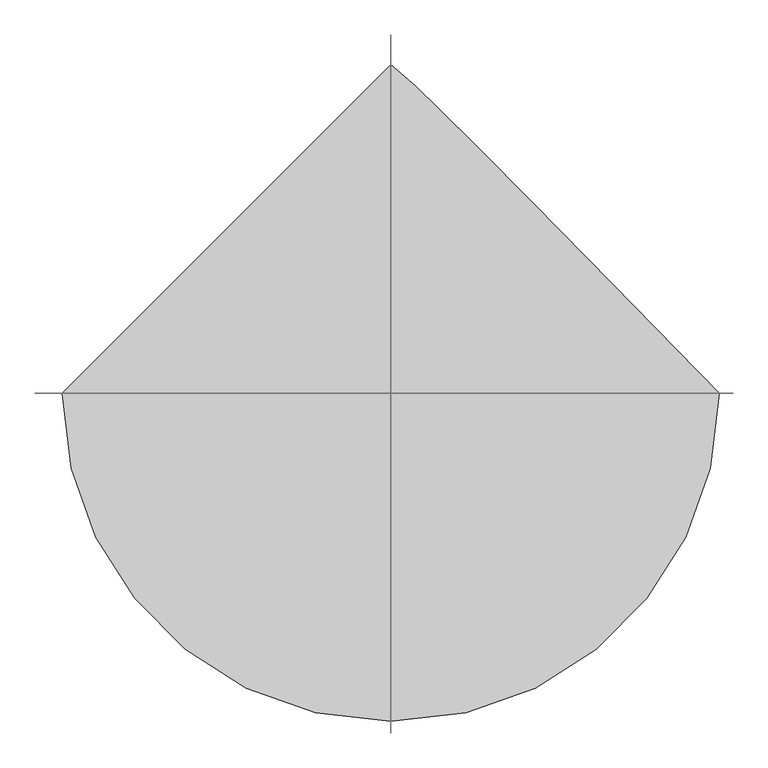
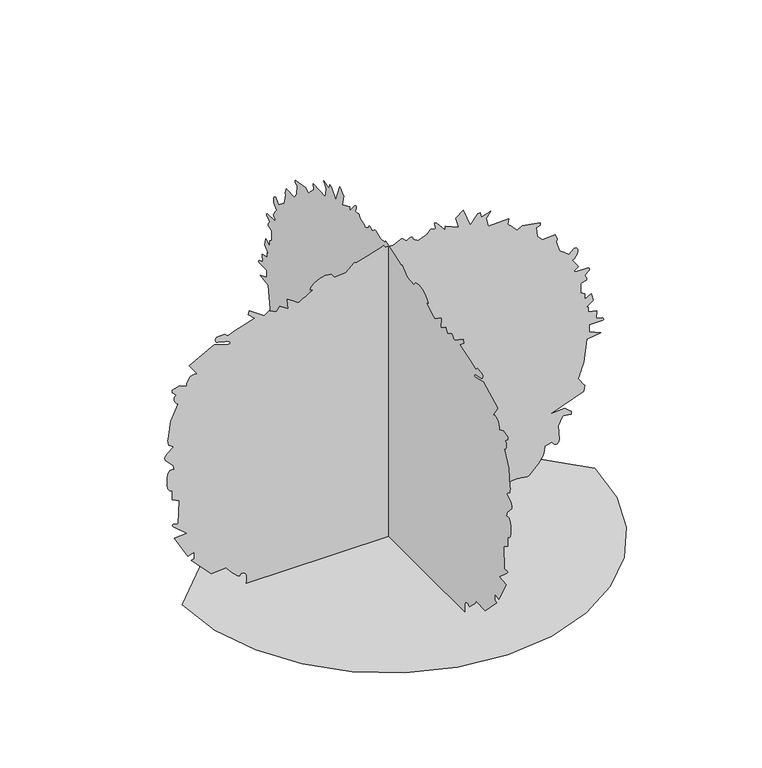
"""IFC4 building model written with IfcOpenShell, lengths in millimetres: proxy geometry, holly 26751 : holly 26751."""

import ifcopenshell
import ifcopenshell.guid

model = None  # the IFC model being written
_history = None  # IfcOwnerHistory: only IFC2X3 demands one
_inside = {}  # id of a spatial element -> (the spatial element, [elements in it])
_under = {}  # id of a project, library or spatial element -> (it, [spatial elements below it])
_declared = {}  # id of a project -> (the project, [libraries it declares])
_typed = {}  # id of a type object -> (the type object, [elements of that type])
_made_of = {}  # id of a material, layer set ... -> (it, [elements and type objects made of it])


def new_model(schema):
    """Start an empty IFC model of exactly this schema.

    Asked for "IFC4X3", IfcOpenShell would pick the latest addendum, in which some entities
    have other attributes; the version numbers below select the first issue.
    IFC2X3 requires an IfcOwnerHistory on every rooted entity: one is made here for all.
    """
    global model, _history
    if schema == "IFC4X3":
        model = ifcopenshell.file(schema_version=(4, 3, 0, 0))
    else:
        model = ifcopenshell.file(schema=schema)
    _inside.clear()
    _under.clear()
    _declared.clear()
    _typed.clear()
    _made_of.clear()
    _history = None
    if model.schema == "IFC2X3":
        org = make("IfcOrganization", Name="unknown")
        user = make(
            "IfcPersonAndOrganization",
            ThePerson=make("IfcPerson", FamilyName="unknown"),
            TheOrganization=org,
        )
        app = make(
            "IfcApplication",
            ApplicationDeveloper=org,
            Version="unknown",
            ApplicationFullName="unknown",
            ApplicationIdentifier="unknown",
        )
        _history = make(
            "IfcOwnerHistory",
            OwningUser=user,
            OwningApplication=app,
            ChangeAction="ADDED",
            CreationDate=0,
        )
    return model


def make(cls, **values):
    """One entity of the class cls with the attributes given. An attribute that is None is left unset."""
    return model.create_entity(
        cls, **{name: value for name, value in values.items() if value is not None}
    )


def rooted(cls, **values):
    """An entity with a GlobalId (a new one), such as an element, a storey or a relation."""
    return make(cls, GlobalId=ifcopenshell.guid.new(), OwnerHistory=_history, **values)


def si_unit(unit_type, name, prefix=None):
    """IfcSIUnit, for example si_unit("LENGTHUNIT", "METRE", prefix="MILLI")."""
    return make("IfcSIUnit", UnitType=unit_type, Prefix=prefix, Name=name)


def assignment(units):
    """IfcUnitAssignment: the units of a project."""
    return None if units is None else make("IfcUnitAssignment", Units=units)


def point(xyz):
    """IfcCartesianPoint."""
    return None if xyz is None else make("IfcCartesianPoint", Coordinates=xyz)


def direction(xyz):
    """IfcDirection."""
    return None if xyz is None else make("IfcDirection", DirectionRatios=xyz)


def frame(location, z_axis=None, x_axis=None):
    """IfcAxis2Placement3D, a coordinate frame: its origin and axes. An axis left out is left unset."""
    return make(
        "IfcAxis2Placement3D",
        Location=point(location),
        Axis=direction(z_axis),
        RefDirection=direction(x_axis),
    )


def origin():
    """The frame at (0, 0, 0) with its axes left unset."""
    return frame((0.0, 0.0, 0.0))


def place(relative_to, where):
    """IfcLocalPlacement: puts the frame where relative to a parent placement (None: the world)."""
    return make(
        "IfcLocalPlacement", PlacementRelTo=relative_to, RelativePlacement=where
    )


def context(
    kind, dimensions, precision=None, world=None, true_north=None, identifier=None
):
    """IfcGeometricRepresentationContext, for example the 3D "Model" context."""
    return make(
        "IfcGeometricRepresentationContext",
        ContextIdentifier=identifier,
        ContextType=kind,
        CoordinateSpaceDimension=dimensions,
        Precision=precision,
        WorldCoordinateSystem=world,
        TrueNorth=true_north,
    )


def project(units=None, contexts=None):
    """IfcProject with its units and contexts."""
    return rooted(
        "IfcProject",
        Name="project",
        RepresentationContexts=contexts,
        UnitsInContext=assignment(units),
    )


def spatial(cls, under=None, at=None, **own):
    """A site, building, storey or space (cls), placed at a placement, below another one or the project."""
    s = rooted(cls, ObjectPlacement=at, **own)
    if under is not None:
        _under.setdefault(under.id(), (under, []))[1].append(s)
    return s


def point_list(points):
    """IfcCartesianPointList2D or 3D."""
    cls = (
        "IfcCartesianPointList2D" if len(points[0]) == 2 else "IfcCartesianPointList3D"
    )
    return make(cls, CoordList=points)


def triangles(points, corners, closed=None, point_numbers=None):
    """IfcTriangulatedFaceSet: each triangle names its three corners, points numbered from 1."""
    return make(
        "IfcTriangulatedFaceSet",
        Coordinates=point_list(points),
        Closed=closed,
        CoordIndex=corners,
        PnIndex=point_numbers,
    )


def shape(context_of_items, identifier, shape_type, items):
    """IfcShapeRepresentation: the items that make up one representation, for example the "Body"."""
    return make(
        "IfcShapeRepresentation",
        ContextOfItems=context_of_items,
        RepresentationIdentifier=identifier,
        RepresentationType=shape_type,
        Items=items,
    )


def source(mapping_origin, context_of_items, identifier, shape_type, items):
    """IfcRepresentationMap: a shape defined once, which mapped items show again and again."""
    return make(
        "IfcRepresentationMap",
        MappingOrigin=mapping_origin,
        MappedRepresentation=shape(context_of_items, identifier, shape_type, items),
    )


def transform(
    local_origin,
    x_axis=None,
    y_axis=None,
    z_axis=None,
    scale=None,
    scale2=None,
    scale3=None,
    uniform=True,
):
    """IfcCartesianTransformationOperator3D, or its non-uniform kind. x_axis, y_axis, z_axis: its Axis1, 2, 3."""
    if uniform:
        return make(
            "IfcCartesianTransformationOperator3D",
            Axis1=direction(x_axis),
            Axis2=direction(y_axis),
            LocalOrigin=point(local_origin),
            Scale=scale,
            Axis3=direction(z_axis),
        )
    return make(
        "IfcCartesianTransformationOperator3DnonUniform",
        Axis1=direction(x_axis),
        Axis2=direction(y_axis),
        LocalOrigin=point(local_origin),
        Scale=scale,
        Axis3=direction(z_axis),
        Scale2=scale2,
        Scale3=scale3,
    )


def mapped(mapping_source, mapping_target):
    """IfcMappedItem: shows the shape of a source again, moved by a transform."""
    return make(
        "IfcMappedItem", MappingSource=mapping_source, MappingTarget=mapping_target
    )


def made_of(thing, what):
    """Note that an element or type object is made of a material, layer set ...; save() writes the relation."""
    if what is not None:
        _made_of.setdefault(what.id(), (what, []))[1].append(thing)
    return thing


def element(
    cls,
    number,
    at=None,
    inside=None,
    cuts=None,
    type_object=None,
    material=None,
    context=None,
    identifier="Body",
    shape_type=None,
    held_by="IfcProductDefinitionShape",
    body=None,
    shapes=None,
    **own,
):
    """One element of the class cls, such as IfcWall. Its Tag is "e" and its number.

    at: its placement. inside: the storey or other place that contains it. cuts: it is an
    opening in that element (IfcRelVoidsElement). A single representation is given by context,
    identifier, shape_type and body (its items); several are given by shapes. held_by: the class
    of the entity that holds the representations. save() writes the other relations.
    """
    e = rooted(cls, Tag="e%d" % number, ObjectPlacement=at, **own)
    if body is not None:
        shapes = [shape(context, identifier, shape_type, body)]
    if shapes is not None:
        e.Representation = make(held_by, Representations=shapes)
    if inside is not None:
        _inside.setdefault(inside.id(), (inside, []))[1].append(e)
    if cuts is not None:
        rooted(
            "IfcRelVoidsElement", RelatingBuildingElement=cuts, RelatedOpeningElement=e
        )
    if type_object is not None:
        _typed.setdefault(type_object.id(), (type_object, []))[1].append(e)
    return made_of(e, material)


def aggregate(whole, parts):
    """IfcRelAggregates: a whole, such as a stair, and the parts it consists of."""
    return rooted("IfcRelAggregates", RelatingObject=whole, RelatedObjects=parts)


def save(model, path):
    """Write the relations noted so far, then the file.

    IfcRelAggregates (storeys below a building ...), IfcRelContainedInSpatialStructure (elements
    in a storey), IfcRelDefinesByType, IfcRelAssociatesMaterial and IfcRelDeclares: one each for
    every whole, place, type object, material and project.
    """
    for whole, parts in _under.values():
        aggregate(whole, parts)
    for where, things in _inside.values():
        rooted(
            "IfcRelContainedInSpatialStructure",
            RelatedElements=things,
            RelatingStructure=where,
        )
    for kind, things in _typed.values():
        rooted("IfcRelDefinesByType", RelatedObjects=things, RelatingType=kind)
    for what, things in _made_of.values():
        rooted("IfcRelAssociatesMaterial", RelatedObjects=things, RelatingMaterial=what)
    for by, libraries in _declared.values():
        rooted("IfcRelDeclares", RelatingContext=by, RelatedDefinitions=libraries)
    model.write(path)


def entourage_54f20335(model_context):
    return source(origin(), model_context, "Body", "Tessellation", [
        triangles([(-823.0310858, 0.0, 7.21e-05), (-801.2709314, -188.5840741, 7.21e-05), (-739.3050917, -361.7670897, 7.21e-05), (-642.0891506, -514.5912643, 7.21e-05), (-514.5912643, -642.0891506, 7.21e-05), (-361.7670897, -739.3050917, 7.21e-05), (-188.5840741, -801.2709314, 7.21e-05), (3.6e-05, -823.0310858, 7.21e-05), (188.5840741, -801.2709314, 7.21e-05), (361.7670897, -739.3050917, 7.21e-05), (514.5912643, -642.0891506, 7.21e-05), (642.0891506, -514.5912643, 7.21e-05), (739.3050917, -361.7670897, 7.21e-05), (801.2709314, -188.5838197, 7.21e-05), (823.0310858, 7.2e-05, 7.21e-05), (555.5640178, 274.3555465, 7.21e-05), (357.2763754, 476.3515926, 7.21e-05), (216.6411551, 618.0454874, 7.21e-05), (122.1254853, 711.5022102, 7.21e-05), (62.2002777, 768.7766939, 7.21e-05), (25.3349997, 801.933827, 7.21e-05), (-0.0001079, 823.0310858, 7.21e-05), (0.0, 364.688096, 1198.1839863), (0.0, 394.9268025, 1235.9816792), (0.0, 406.2653546, 1235.9816792), (0.0, 410.0448841, 1217.0841408), (0.0, 447.8426133, 1228.4226929), (0.0, 428.9450386, 1205.7430452), (0.0, 436.5040612, 1167.9452797), (0.0, 519.6585786, 1171.727389), (0.0, 515.8790491, 1149.0476686), (0.0, 517.7484844, 1147.6176687), (0.0, 521.9039357, 1143.7644882), (0.0, 527.6798913, 1138.1510954), (0.0, 534.4109121, 1131.4328281), (0.0, 541.4314502, 1124.2699659), (0.0, 548.0735593, 1117.3230789), (0.0, 553.6768147, 1111.2499758), (0.0, 572.5743894, 1122.5885279), (0.0, 644.390391, 1111.2499758), (0.0, 644.390391, 1099.9114237), (0.0, 629.2722731, 1096.1318579), (0.0, 633.0517662, 1058.334165), (0.0, 651.9493773, 1035.6544447), (0.0, 704.8677315, 1039.4340105), (0.0, 712.4267904, 1016.7569063), (0.0, 708.6472973, 1009.1953039), (0.0, 719.9858494, 967.6180452), (0.0, 726.0208735, 963.2238367), (0.0, 732.9550432, 957.9761919), (0.0, 740.1179054, 952.4085085), (0.0, 746.8488899, 947.0389961), (0.0, 752.4800869, 942.3932768), (0.0, 756.345912, 938.9998793), (0.0, 757.7835423, 937.3818821), (0.0, 780.4607191, 956.2794931), (0.0, 789.1297394, 953.9172827), (0.0, 793.4883396, 947.7375), (0.0, 794.1741262, 939.096385), (0.0, 791.8195461, 929.3580259), (0.0, 787.0672199, 919.8812788), (0.0, 780.5495945, 912.0225288), (0.0, 772.9016602, 907.1431755), (0.0, 774.118301, 904.8622828), (-2e-07, 781.5884846, 895.1949949), (-2e-07, 794.0852509, 877.4074179), (0.0, 795.5813078, 873.1249758), (0.0, 794.0014624, 870.5621235), (0.0, 782.7695171, 862.2893), (0.0, 780.9686823, 860.2395704), (0.0, 780.4607191, 858.0068579), (2e-07, 785.7515299, 855.1773067), (-2e-07, 836.9528378, 853.0538898), (0.0, 840.9380596, 850.4453281), (1e-07, 841.2580982, 846.6200529), (1e-07, 839.7290491, 843.1504246), (0.0, 822.0405212, 827.768224), (3e-07, 829.193137, 816.4016939), (5e-07, 829.9424372, 812.9472536), (7e-07, 829.5335232, 809.4446331), (7e-07, 829.7087305, 806.8944981), (6e-07, 827.806303, 805.096134), (0.0, 810.7247875, 799.7900625), (0.0, 806.9198599, 797.5295174), (0.0, 806.9198599, 759.7317518), (0.0, 822.0405212, 748.3931997), (0.0, 822.0405212, 725.7135521), (0.0, 848.4971186, 740.8341408), (0.0, 856.0561775, 710.5954342), (0.0, 829.5995075, 691.6952797), (0.0, 837.1585665, 687.9157866), (0.0, 837.1585665, 669.0181755), (0.0, 871.1767662, 661.4591892), (0.0, 867.3972731, 631.2204826), (-4e-07, 892.5458107, 622.5819111), (-3e-07, 895.9697296, 619.724382), (0.0, 897.6334362, 616.1023647), (3e-07, 893.5719835, 613.0467373), (0.0, 840.9380596, 612.3203281), (0.0, 840.9380596, 582.084165), (0.0, 886.2948841, 563.1840105), (0.0, 829.5995075, 555.6249879), (0.0, 818.258412, 461.1319184), (0.0, 815.0631128, 451.4214646), (0.0, 811.202302, 440.3089889), (0.0, 807.0646185, 428.8484965), (0.0, 803.043861, 418.0966819), (0.0, 799.5284506, 409.1101665), (0.0, 796.9122585, 402.9455718), (0.0, 795.5813078, 400.6545053), (0.0, 820.5621958, 364.3553764), (0.0, 822.0405212, 362.856776), (0.0, 818.258412, 340.1796355), (-1.2e-06, 685.9676497, 291.7393147), (0.0, 742.6629536, 294.8203221), (0.0, 767.2044062, 273.0017229), (0.0, 769.1220943, 272.1432179), (0.0, 769.1220943, 260.8046476), (0.0, 735.1038946, 264.5841771), (0.0, 716.2062836, 230.5654505), (6e-07, 720.5065298, 170.5523622), (4e-07, 718.0097345, 161.443416), (0.0, 712.4267904, 154.9702283), (1e-07, 708.1747971, 154.6016643), (1e-07, 704.4080212, 155.6534715), (1e-07, 701.0399855, 157.7794682), (0.0, 689.7471428, 170.0893091), (0.0, 663.2904728, 162.5297596), (0.0, 661.3549805, 143.989803), (0.0, 655.9651205, 127.1831253), (0.0, 637.3164768, 97.7790698), (0.0, 599.0335665, 60.4761278), (0.0, 593.0747369, 58.4339696), (0.0, 555.4065419, 64.3069578), (0.0, 530.3748576, 63.9444981), (0.0, 505.6580887, 55.865013), (0.0, 484.5938948, 35.9298222), (0.0, 470.5222973, 0.0), (1.9e-06, -527.336998, 0.3946068), (1.9e-06, -526.7324927, 3.4093656), (1.8e-06, -525.6326689, 11.1126779), (1.6e-06, -525.1043581, 21.4932261), (1.4e-06, -526.211776, 32.5396858), (1.3e-06, -530.0217905, 42.240454), (1.2e-06, -537.6011244, 48.584103), (1.1e-06, -550.0141022, 49.5597157), (1.1e-06, -552.9884482, 42.5897014), (9e-07, -560.6973527, 44.5830936), (4e-07, -583.0569617, 64.6592528), (2e-07, -594.0755116, 77.3417272), (1e-07, -602.5667084, 88.1867683), (0.0, -606.7119859, 94.4940959), (0.0, -667.1868193, 90.7143212), (0.0, -746.5618435, 173.8690929), (0.0, -735.2232914, 177.6488585), (0.0, -735.2232914, 204.1070183), (0.0, -761.6799614, 196.547487), (0.0, -814.5983156, 291.0408108), (0.0, -765.461998, 294.8203221), (-1e-07, -818.4387789, 340.9873624), (0.0, -822.1573019, 347.7386945), (-3e-07, -820.8568726, 350.2888295), (-4e-07, -818.2406805, 351.2819738), (0.0, -799.4776543, 347.7386945), (0.0, -795.6981611, 442.2317639), (0.0, -822.1573019, 457.352389), (0.0, -822.1573019, 495.1475747), (0.0, -832.8634071, 498.9677267), (1e-07, -839.8280983, 508.9931322), (2e-07, -843.5822296, 523.0672731), (5e-07, -843.58986, 554.7486969), (7e-07, -840.9076109, 568.0481031), (9e-07, -837.1458492, 576.780637), (6e-07, -835.3424709, 579.5238198), (4e-07, -832.4240444, 581.3678933), (1e-07, -824.7836678, 582.9223406), (0.0, -814.5983156, 582.084165), (0.0, -818.9670897, 599.2621862), (0.0, -850.1633686, 632.368523), (0.0, -852.289329, 643.412471), (0.0, -843.1225193, 657.5323214), (0.0, -818.3778088, 676.5772345), (0.0, -819.0966602, 678.065661), (0.0, -834.2578714, 690.2068531), (0.0, -837.2754198, 691.6952797), (0.0, -841.0549129, 714.375), (0.0, -838.9950096, 718.3525915), (0.0, -829.7163609, 789.9704584), (0.0, -799.4776543, 854.2273647), (0.0, -805.1469303, 855.9037886), (0.0, -809.7265926, 860.3360762), (0.0, -812.954884, 866.6098938), (0.0, -814.5627073, 873.8234797), (0.0, -814.2909216, 881.0700577), (0.0, -811.8703571, 887.4378376), (0.0, -807.0392567, 892.0251303), (0.0, -807.4354534, 892.8607624), (0.0, -812.0837162, 897.9737497), (0.0, -820.8492422, 906.3049999), (0.0, -822.1573019, 907.1431755), (0.0, -822.1573019, 918.4817276), (0.0, -791.9185953, 926.0407866), (0.0, -790.6511581, 925.0044399), (0.0, -777.4609749, 918.7560568), (0.0, -765.461998, 914.7022345), (0.0, -764.4104633, 924.481216), (0.0, -761.392915, 934.0036726), (0.0, -756.6100674, 942.5457384), (0.0, -750.2651785, 949.3884893), (0.0, -742.5613609, 953.8080597), (0.0, -733.6992565, 955.0856707), (0.0, -723.8821959, 952.5), (0.0, -754.1209024, 997.8567518), (0.0, -655.8482672, 1050.775106), (7e-07, -598.9294304, 1033.6808733), (5e-07, -592.5108541, 1034.3742903), (5e-07, -591.6802726, 1035.5045992), (4e-07, -591.6421935, 1037.1784796), (3e-07, -592.2771838, 1039.2003038), (2e-07, -595.0864237, 1043.5360857), (0.0, -599.1504198, 1046.9930695), (0.0, -613.793494, 1050.1477461), (0.0, -641.0578909, 1056.558692), (0.0, -644.5071716, 1058.334165), (1e-07, -646.8948166, 1060.1705355), (1e-07, -648.7185425, 1062.5454632), (1e-07, -649.9529875, 1065.3064138), (1e-07, -650.5574564, 1068.3061581), (0.0, -650.5041166, 1071.3923069), (0.0, -649.7573599, 1074.4174129), (0.0, -648.2892809, 1077.2317034), (-2e-07, -645.2513849, 1079.2662449), (0.0, -614.2710085, 1081.0112692), (0.0, -603.3617543, 1070.5744062), (0.0, -602.9299493, 1069.6727171), (0.0, -567.8931707, 1083.2083735), (0.0, -547.3801423, 1090.3508154), (0.0, -493.3187983, 1107.47041), (0.0, -519.7754319, 1130.1475868), (0.0, -515.9959024, 1145.2681755), (0.0, -455.5210327, 1103.6909168), (0.0, -436.6209146, 1118.8089621), (0.0, -406.382208, 1103.6909168), (0.0, -405.4525772, 1104.4097683), (0.0, -396.018996, 1119.5709795), (0.0, -395.0436559, 1122.5885279), (0.0, -361.0254198, 1099.9114237), (0.0, -365.1427557, 1139.9113077), (0.0, -364.8049493, 1141.4886824), (0.0, -342.607903, 1128.2831657), (0.0, -319.4481611, 1111.2499758), (0.0, -309.9866747, 1116.2283783), (0.0, -299.4278897, 1122.1567228), (0.0, -288.7040166, 1128.4457285), (0.0, -278.7446681, 1134.4934698), (0.0, -270.4795113, 1139.7106659), (0.0, -264.8381769, 1143.5003328), (0.0, -262.752839, 1145.2681755), (0.0, -273.3471778, 1149.5912401), (0.0, -269.0418629, 1159.9925674), (0.0, -254.1727123, 1172.6036436), (0.0, -233.0803043, 1183.5662739), (0.0, -210.0991489, 1189.0196474), (0.0, -189.5657729, 1185.1004826), (0.0, -175.8177748, 1167.9452797), (0.0, -130.4607414, 1171.727389), (0.0, -96.4430322, 1201.9634794), (0.0, -95.7204019, 1201.8238077), (0.0, -89.6495515, 1198.8037886), (0.0, -88.8834827, 1198.1839863), (0.0, -39.7464248, 1213.3046476), (0.0, 20.7297008, 1232.2022587), (0.0, 21.3109812, 1231.442712), (0.0, 21.9957141, 1230.3632721), (0.0, 22.7131871, 1229.0906754), (0.0, 23.3937551, 1227.7547104), (0.0, 23.9666262, 1226.4821136), (0.0, 24.3619509, 1225.4026737), (0.0, 24.5094506, 1224.6431271), (0.0, 58.527187, 1220.8637066), (0.0, 88.228163, 1235.3035229), (0.0, 92.5451506, 1235.9816792), (-1e-07, 95.4963785, 1234.686264), (0.0, 109.5573117, 1221.6231079), (0.0, 111.4440243, 1220.8637066), (0.0, 122.4526365, 1227.7801449), (0.0, 128.2821862, 1229.7790054), (0.0, 133.4833494, 1229.5072197), (0.0, 137.0317248, 1225.6972778), (0.0, 137.9024383, 1217.0841408), (0.0, 140.9202138, 1215.7049372), (0.0, 144.3867991, 1213.9269207), (0.0, 147.9687116, 1211.9380886), (0.0, 151.3339586, 1209.9340685), (0.0, 154.1492937, 1208.1052557), (0.0, 156.0827331, 1206.6447344), (0.0, 156.801312, 1205.7430452), (0.0, 162.3971732, 1208.1433348), (0.0, 169.0263289, 1210.9119158), (0.0, 176.0290991, 1213.7770752), (0.0, 182.746894, 1216.4745123), (0.0, 188.5205787, 1218.7325867), (0.0, 192.691, 1220.2871429), (0.0, 194.5987869, 1220.8637066), (0.0, 205.4400219, 1235.8141022), (0.0, 205.9381202, 1235.9816792), (0.0, 208.316318, 1235.3645657), (0.0, 227.1496525, 1232.3444012), (0.0, 228.6167504, 1232.2022587), (1e-07, 223.3642912, 1249.3599323), (1e-07, 222.9002389, 1253.4188416), (1e-07, 223.3033211, 1256.642046), (0.0, 224.8369848, 1258.6613995), (-3e-07, 231.8636453, 1254.2900093), (0.0, 264.139673, 1215.5067661), (0.0, 266.4129717, 1213.3046476), (0.0, 266.4129717, 1228.4226929), (0.0, 319.3313441, 1205.7430452), (0.0, 307.9927557, 1247.3202312), (0.0, 338.2289188, 1269.9999516), (325.0107576, -3.63e-05, 1198.1839863), (355.2494642, -3.85e-05, 1235.9816792), (366.5880163, -3.85e-05, 1235.9816792), (370.3675458, -3.74e-05, 1217.0841408), (408.165275, -3.81e-05, 1228.4226929), (389.2677003, -3.67e-05, 1205.7430452), (396.8267229, -3.44e-05, 1167.9452797), (479.9812403, -3.47e-05, 1171.727389), (476.2017108, -3.33e-05, 1149.0476686), (478.0711461, -3.32e-05, 1147.6176687), (482.2265974, -3.3e-05, 1143.7644882), (488.002553, -3.27e-05, 1138.1510954), (494.7335738, -3.23e-05, 1131.4328281), (501.7515684, -3.18e-05, 1124.2699659), (508.396221, -3.14e-05, 1117.3230789), (513.9994763, -3.11e-05, 1111.2499758), (532.897051, -3.17e-05, 1122.5885279), (604.7130163, -3.11e-05, 1111.2499758), (604.7130163, -3.04e-05, 1099.9114237), (589.5949347, -3.02e-05, 1096.1318579), (593.3744642, -2.79e-05, 1058.334165), (612.2720753, -2.66e-05, 1035.6544447), (665.187886, -2.68e-05, 1039.4340105), (672.7494884, -2.54e-05, 1016.7569063), (668.9699226, -2.5e-05, 1009.1953039), (680.3084747, -2.25e-05, 967.6180452), (686.3434988, -2.22e-05, 963.2238367), (693.2777412, -2.19e-05, 957.9761919), (700.4405308, -2.16e-05, 952.4085085), (707.1715153, -2.13e-05, 947.0389961), (712.8027122, -2.1e-05, 942.3932768), (716.66861, -2.08e-05, 938.9998793), (718.1062403, -2.07e-05, 937.3818821), (740.7833445, -2.18e-05, 956.2794931), (749.4523647, -2.17e-05, 953.9172827), (753.8110376, -2.13e-05, 947.7375), (754.4942808, -2.08e-05, 939.096385), (752.1422441, -2.02e-05, 929.3580259), (747.3899179, -1.97e-05, 919.8812788), (740.8722198, -1.92e-05, 912.0225288), (733.2242855, -1.89e-05, 907.1431755), (734.440999, -1.87e-05, 904.8622828), (741.9111099, -1.8e-05, 895.1949949), (754.4078762, -1.69e-05, 877.4074179), (755.9040058, -1.69e-05, 873.1249758), (754.3240877, -1.68e-05, 870.5621235), (743.0922152, -1.62e-05, 862.2893), (741.2913803, -1.61e-05, 860.2395704), (740.7833445, -1.6e-05, 858.0068579), (746.0741552, -1.6e-05, 855.1773067), (797.2754631, -1.54e-05, 853.0538898), (801.2607576, -1.55e-05, 850.4453281), (801.5807962, -1.54e-05, 846.6200529), (800.0516745, -1.52e-05, 843.1504246), (782.3606031, -1.42e-05, 827.768224), (789.5157623, -1.38e-05, 816.4016939), (790.2650625, -1.38e-05, 812.9472536), (789.8561485, -1.38e-05, 809.4446331), (790.0314285, -1.36e-05, 806.8944981), (788.1289284, -1.34e-05, 805.096134), (771.0474855, -1.25e-05, 799.7900625), (767.2425579, -1.24e-05, 797.5295174), (767.2425579, -1.01e-05, 759.7317518), (782.3606031, -9.4e-06, 748.3931997), (782.3606031, -8.1e-06, 725.7135521), (808.8198166, -9e-06, 740.8341408), (816.3788029, -7.2e-06, 710.5954342), (789.9222055, -6.1e-06, 691.6952797), (797.4812645, -5.8e-06, 687.9157866), (797.4812645, -4.7e-06, 669.0181755), (831.4994642, -4.3e-06, 661.4591892), (827.7198984, -2.5e-06, 631.2204826), (852.8684361, -1.6e-06, 622.5819111), (856.292355, -1.5e-06, 619.724382), (857.9560616, -1.6e-06, 616.1023647), (853.8946089, -1.7e-06, 613.0467373), (801.2607576, -1.3e-06, 612.3203281), (801.2607576, 5e-07, 582.084165), (846.6175095, 1.6e-06, 563.1840105), (789.9222055, 2e-06, 555.6249879), (778.58111, 7.7e-06, 461.1319184), (775.3857382, 8.3e-06, 451.4214646), (771.525, 8.9e-06, 440.3089889), (767.3873165, 9.6e-06, 428.8484965), (763.3664864, 1.02e-05, 418.0966819), (759.8511486, 1.08e-05, 409.1101665), (757.2349566, 1.11e-05, 402.9455718), (755.9040058, 1.13e-05, 400.6545053), (780.8823503, 1.34e-05, 364.3553764), (782.3606031, 1.35e-05, 362.856776), (778.58111, 1.49e-05, 340.1796355), (646.290275, 1.9e-05, 291.7393147), (702.9855789, 1.76e-05, 294.8203221), (727.5271042, 1.89e-05, 273.0017229), (729.4447924, 1.89e-05, 272.1432179), (729.4447924, 1.96e-05, 260.8046476), (695.4265926, 1.94e-05, 264.5841771), (676.5289816, 2.14e-05, 230.5654505), (680.8292278, 2.44e-05, 170.5523622), (678.3323599, 2.51e-05, 161.4436704), (672.7494884, 2.59e-05, 154.9702283), (668.4974951, 2.59e-05, 154.6016643), (664.7306465, 2.58e-05, 155.6534715), (661.3626108, 2.56e-05, 157.7794682), (650.0697681, 2.5e-05, 170.0893091), (623.6106274, 2.55e-05, 162.5297596), (621.675135, 2.66e-05, 143.989803), (616.2852751, 2.76e-05, 127.1833797), (597.6391022, 2.93e-05, 97.7790698), (559.3562282, 3.16e-05, 60.4761278), (553.3948551, 3.17e-05, 58.4342239), (515.7292036, 3.13e-05, 64.3069578), (490.6975193, 3.14e-05, 63.9444981), (465.9807504, 3.18e-05, 55.8652674), (444.9165565, 3.3e-05, 35.9298222), (430.844959, 3.52e-05, 5e-05), (-567.0143363, 3.32e-05, 0.3946575), (-566.409831, 3.31e-05, 3.4094164), (-565.3100072, 3.27e-05, 11.1127279), (-564.7816964, 3.23e-05, 21.4932761), (-565.8891143, 3.18e-05, 32.5396858), (-569.6991288, 3.14e-05, 42.240454), (-577.2784627, 3.11e-05, 48.584103), (-589.6914405, 3.11e-05, 49.5597157), (-592.6657866, 3.16e-05, 42.5897014), (-600.374691, 3.16e-05, 44.5830936), (-622.7343, 3.09e-05, 64.6592528), (-633.7528135, 3.03e-05, 77.3417272), (-642.244083, 2.98e-05, 88.1867683), (-646.3893242, 2.95e-05, 94.4940959), (-706.8641939, 2.98e-05, 90.7143212), (-786.2392181, 2.48e-05, 173.8690929), (-774.900666, 2.46e-05, 177.6488585), (-774.900666, 2.3e-05, 204.1072726), (-801.3598068, 2.35e-05, 196.5477413), (-854.2756176, 1.78e-05, 291.0408108), (-805.1393, 1.76e-05, 294.8203221), (-858.1160809, 1.5e-05, 340.9873624), (-861.8346766, 1.44e-05, 347.7386945), (-860.5341745, 1.46e-05, 350.2888295), (-857.9179825, 1.46e-05, 351.2819738), (-839.1550289, 1.44e-05, 347.7386945), (-835.3754631, 8.8e-06, 442.2317639), (-861.8346766, 7.9e-06, 457.352389), (-861.8346766, 5.7e-06, 495.1475747), (-872.5433252, 5.4e-06, 498.9677267), (-879.5054729, 4.7e-06, 508.9931322), (-883.2595316, 3.8e-06, 523.0672731), (-883.2671619, 1.6e-06, 554.7486969), (-880.5874563, 6e-07, 568.0481031), (-876.8257673, -2e-07, 576.780637), (-875.0197729, 0.0, 579.5238198), (-872.1013464, 1e-07, 581.3678933), (-864.4610424, 3e-07, 582.9223406), (-854.2756176, 5e-07, 582.084165), (-858.6443916, -6e-07, 599.2621862), (-889.8406706, -2.5e-06, 632.368523), (-891.9667036, -3.2e-06, 643.412471), (-882.8023647, -4e-06, 657.5323214), (-858.0551834, -5.2e-06, 676.5772345), (-858.7739622, -5.2e-06, 678.065661), (-873.9352461, -6e-06, 690.2068531), (-876.9527218, -6.1e-06, 691.6952797), (-880.734831, -7.4e-06, 714.375), (-878.6723116, -7.7e-06, 718.3525915), (-869.3937355, -1.19e-05, 789.9704584), (-839.1550289, -1.57e-05, 854.2273647), (-844.824305, -1.58e-05, 855.9037886), (-849.4064381, -1.61e-05, 860.3360762), (-852.6322586, -1.65e-05, 866.6098938), (-854.240082, -1.69e-05, 873.8234797), (-853.9682962, -1.73e-05, 881.0700577), (-851.5476591, -1.77e-05, 887.4378376), (-846.7165586, -1.8e-05, 892.0225868), (-847.1128281, -1.81e-05, 892.8607624), (-851.7610182, -1.84e-05, 897.9737497), (-860.5265442, -1.89e-05, 906.3049999), (-861.8346766, -1.89e-05, 907.1431755), (-861.8346766, -1.96e-05, 918.4817276), (-831.59597, -2e-05, 926.0407866), (-830.3285328, -2e-05, 925.0044399), (-817.1382769, -1.96e-05, 918.7560568), (-805.1393, -1.94e-05, 914.7022345), (-804.0877653, -1.99e-05, 924.481216), (-801.0702169, -2.05e-05, 934.0036726), (-796.287442, -2.1e-05, 942.5457384), (-789.9424805, -2.14e-05, 949.3884893), (-782.2386629, -2.17e-05, 953.8080597), (-773.3766312, -2.18e-05, 955.0856707), (-763.5620413, -2.16e-05, 952.5), (-793.7982044, -2.43e-05, 997.8567518), (-695.5256418, -2.75e-05, 1050.775106), (-638.606805, -2.72e-05, 1033.6808733), (-632.1882288, -2.7e-05, 1034.3742903), (-631.3576109, -2.7e-05, 1035.5045992), (-631.3195318, -2.71e-05, 1037.1784796), (-631.9545221, -2.71e-05, 1039.2003038), (-634.7637257, -2.72e-05, 1043.5360857), (-638.8277218, -2.72e-05, 1046.9930695), (-653.4708687, -2.74e-05, 1050.1477461), (-680.7351929, -2.78e-05, 1056.558692), (-684.1870897, -2.79e-05, 1058.334165), (-686.5721186, -2.81e-05, 1060.1705355), (-688.3983879, -2.83e-05, 1062.5454632), (-689.6302895, -2.84e-05, 1065.3064138), (-690.234831, -2.86e-05, 1068.3061581), (-690.1814913, -2.87e-05, 1071.3923069), (-689.4347345, -2.89e-05, 1074.4174129), (-687.9665829, -2.9e-05, 1077.2317034), (-684.9287596, -2.9e-05, 1079.2637741), (-653.9483831, -2.93e-05, 1081.0112692), (-643.0390926, -2.86e-05, 1070.5744062), (-642.609831, -2.86e-05, 1069.6727171), (-607.5705091, -2.94e-05, 1083.2083735), (-587.0574806, -2.98e-05, 1090.3508154), (-532.9961366, -3.08e-05, 1107.47041), (-559.4527702, -3.22e-05, 1130.1475868), (-555.6732408, -3.31e-05, 1145.2681755), (-495.198371, -3.06e-05, 1103.6909168), (-476.2982529, -3.15e-05, 1118.8089621), (-446.0620897, -3.06e-05, 1103.6909168), (-445.1299155, -3.07e-05, 1104.4097683), (-435.6963344, -3.16e-05, 1119.5709795), (-434.7209942, -3.17e-05, 1122.5885279), (-400.7027581, -3.04e-05, 1099.9114237), (-404.820094, -3.28e-05, 1139.9113077), (-404.484831, -3.29e-05, 1141.4886824), (-382.2852413, -3.21e-05, 1128.2831657), (-359.1254994, -3.11e-05, 1111.2499758), (-349.664013, -3.14e-05, 1116.2283783), (-339.1052098, -3.17e-05, 1122.1567228), (-328.3813368, -3.21e-05, 1128.4457285), (-318.4220246, -3.25e-05, 1134.4934698), (-310.1568315, -3.28e-05, 1139.7106659), (-304.5180405, -3.3e-05, 1143.5003328), (-302.4301774, -3.31e-05, 1145.2681755), (-313.024498, -3.34e-05, 1149.5912401), (-308.7192012, -3.4e-05, 1159.990024), (-293.8500506, -3.47e-05, 1172.6036436), (-272.7578969, -3.54e-05, 1183.5662739), (-249.7767416, -3.57e-05, 1189.0196474), (-229.2433655, -3.55e-05, 1185.1004826), (-215.4953675, -3.44e-05, 1167.9452797), (-170.1383431, -3.47e-05, 1171.727389), (-136.1206249, -3.65e-05, 1201.9634794), (-135.3979945, -3.65e-05, 1201.8238077), (-129.3271442, -3.63e-05, 1198.8037886), (-128.5610754, -3.63e-05, 1198.1839863), (-79.424022, -3.72e-05, 1213.3046476), (-18.9479168, -3.83e-05, 1232.2022587), (-18.3666376, -3.82e-05, 1231.442712), (-17.6819047, -3.82e-05, 1230.3632721), (-16.9644305, -3.81e-05, 1229.0906754), (-16.2838637, -3.8e-05, 1227.7547104), (-15.7109914, -3.79e-05, 1226.4821136), (-15.3156656, -3.79e-05, 1225.4026737), (-15.1681682, -3.78e-05, 1224.6431271), (18.8496693, -3.76e-05, 1220.8637066), (48.5505749, -3.84e-05, 1235.3035229), (52.8675579, -3.85e-05, 1235.9816792), (55.8187858, -3.84e-05, 1234.686264), (69.8797145, -3.76e-05, 1221.6231079), (71.7664271, -3.76e-05, 1220.8637066), (82.7750438, -3.8e-05, 1227.7801449), (88.6045935, -3.81e-05, 1229.7790054), (93.8057568, -3.81e-05, 1229.5072197), (97.3541321, -3.79e-05, 1225.6972778), (98.2248457, -3.74e-05, 1217.0841408), (101.2426211, -3.73e-05, 1215.7049372), (104.7092064, -3.72e-05, 1213.9269207), (108.291119, -3.71e-05, 1211.9380886), (111.6563659, -3.7e-05, 1209.9340685), (114.471701, -3.68e-05, 1208.1052557), (116.4051495, -3.68e-05, 1206.6447344), (117.1234559, -3.67e-05, 1205.7430452), (122.7195896, -3.68e-05, 1208.1433348), (129.3487362, -3.7e-05, 1210.9119158), (136.3515156, -3.72e-05, 1213.7770752), (143.0693014, -3.73e-05, 1216.4745123), (148.8427226, -3.75e-05, 1218.7325867), (153.013153, -3.76e-05, 1220.2871429), (154.9211942, -3.76e-05, 1220.8637066), (165.7624293, -3.85e-05, 1235.8141022), (166.2605275, -3.85e-05, 1235.9816792), (168.6387254, -3.85e-05, 1235.3645657), (187.4720598, -3.83e-05, 1232.3444012), (188.9389034, -3.83e-05, 1232.2022587), (183.6866986, -3.94e-05, 1249.3599323), (183.2226462, -3.96e-05, 1253.4188416), (183.6257285, -3.98e-05, 1256.642046), (185.1593921, -3.99e-05, 1258.6613995), (192.1860526, -3.93e-05, 1254.2900093), (224.4613173, -3.72e-05, 1215.5067661), (226.7366508, -3.72e-05, 1213.3046476), (226.7366508, -3.81e-05, 1228.4226929), (279.6539876, -3.67e-05, 1205.7430452), (268.3128921, -3.92e-05, 1247.3202312), (298.5515805, -4.05e-05, 1269.9999516)], [[21, 22, 1], [20, 21, 1], [19, 20, 1], [18, 19, 1], [17, 18, 1], [17, 1, 2], [17, 2, 3], [17, 3, 4], [16, 17, 4], [16, 4, 5], [16, 5, 6], [16, 6, 7], [16, 7, 8], [16, 8, 9], [16, 9, 10], [16, 10, 11], [16, 11, 12], [15, 16, 12], [14, 15, 12], [13, 14, 12], [100, 101, 102], [26, 27, 28], [153, 154, 155], [157, 158, 159], [316, 317, 318], [239, 240, 241], [238, 239, 241], [319, 320, 23], [318, 319, 23], [245, 246, 247], [87, 88, 89], [156, 157, 159], [29, 30, 31], [138, 139, 140], [248, 249, 250], [138, 140, 141], [117, 118, 119], [116, 117, 119], [212, 213, 214], [138, 141, 142], [258, 259, 260], [312, 313, 314], [311, 312, 314], [310, 311, 314], [92, 93, 94], [138, 142, 143], [146, 147, 148], [39, 40, 41], [39, 41, 42], [24, 25, 26], [96, 97, 98], [200, 201, 202], [199, 200, 202], [198, 199, 202], [198, 202, 203], [197, 198, 203], [44, 45, 46], [44, 46, 47], [309, 310, 314], [258, 260, 261], [197, 203, 204], [196, 197, 204], [137, 138, 143], [271, 272, 273], [271, 273, 274], [271, 274, 275], [271, 275, 276], [271, 276, 277], [271, 277, 278], [271, 278, 279], [95, 96, 98], [94, 95, 98], [94, 98, 99], [92, 94, 99], [247, 248, 250], [137, 143, 144], [23, 24, 26], [241, 242, 243], [87, 89, 90], [247, 250, 251], [115, 116, 119], [115, 119, 120], [114, 115, 120], [90, 91, 92], [112, 113, 114], [111, 112, 114], [110, 111, 114], [165, 166, 167], [39, 42, 43], [38, 39, 43], [244, 245, 247], [160, 161, 162], [160, 162, 163], [160, 163, 164], [55, 56, 57], [55, 57, 58], [55, 58, 59], [55, 59, 60], [55, 60, 61], [55, 61, 62], [55, 62, 63], [184, 185, 186], [85, 86, 87], [266, 267, 268], [266, 268, 269], [266, 269, 270], [73, 74, 75], [73, 75, 76], [72, 73, 76], [72, 76, 77], [66, 67, 68], [80, 81, 82], [44, 47, 48], [159, 160, 164], [23, 26, 28], [23, 28, 29], [153, 155, 156], [66, 68, 69], [212, 214, 215], [65, 66, 69], [258, 261, 262], [122, 123, 124], [122, 124, 125], [122, 125, 126], [121, 122, 126], [121, 126, 127], [287, 288, 289], [287, 289, 290], [286, 287, 290], [285, 286, 290], [179, 180, 181], [179, 181, 182], [178, 179, 182], [136, 137, 144], [243, 244, 247], [65, 69, 70], [184, 186, 187], [183, 184, 187], [196, 204, 205], [152, 153, 156], [136, 144, 145], [263, 264, 265], [262, 263, 265], [258, 262, 265], [120, 121, 127], [114, 120, 127], [114, 127, 128], [146, 148, 149], [167, 168, 169], [167, 169, 170], [79, 80, 82], [78, 79, 82], [78, 82, 83], [77, 78, 83], [72, 77, 83], [72, 83, 84], [71, 72, 84], [309, 314, 315], [305, 306, 307], [304, 305, 307], [281, 282, 283], [280, 281, 283], [280, 283, 284], [64, 65, 70], [152, 156, 159], [167, 170, 171], [167, 171, 172], [167, 172, 173], [167, 173, 174], [167, 174, 175], [167, 175, 176], [167, 176, 177], [165, 167, 177], [159, 164, 165], [304, 307, 308], [230, 231, 232], [229, 230, 232], [228, 229, 232], [227, 228, 232], [226, 227, 232], [225, 226, 232], [224, 225, 232], [223, 224, 232], [223, 232, 233], [222, 223, 233], [222, 233, 234], [222, 234, 235], [221, 222, 235], [220, 221, 235], [220, 235, 236], [219, 220, 236], [218, 219, 236], [218, 236, 237], [217, 218, 237], [217, 237, 238], [132, 133, 134], [131, 132, 134], [189, 190, 191], [189, 191, 192], [189, 192, 193], [189, 193, 194], [189, 194, 195], [189, 195, 196], [189, 196, 205], [183, 187, 188], [212, 215, 216], [152, 159, 165], [130, 131, 134], [129, 130, 134], [128, 129, 134], [128, 134, 135], [114, 128, 135], [114, 135, 136], [114, 136, 145], [110, 114, 145], [109, 110, 145], [108, 109, 145], [107, 108, 145], [106, 107, 145], [105, 106, 145], [104, 105, 145], [103, 104, 145], [102, 103, 145], [100, 102, 145], [99, 100, 145], [92, 99, 145], [90, 92, 145], [87, 90, 145], [85, 87, 145], [84, 85, 145], [71, 84, 145], [70, 71, 145], [64, 70, 145], [63, 64, 145], [55, 63, 145], [54, 55, 145], [53, 54, 145], [52, 53, 145], [51, 52, 145], [50, 51, 145], [49, 50, 145], [48, 49, 145], [44, 48, 145], [43, 44, 145], [38, 43, 145], [37, 38, 145], [36, 37, 145], [35, 36, 145], [34, 35, 145], [33, 34, 145], [32, 33, 145], [31, 32, 145], [29, 31, 145], [23, 29, 145], [318, 23, 145], [316, 318, 145], [315, 316, 145], [309, 315, 145], [308, 309, 145], [304, 308, 145], [303, 304, 145], [302, 303, 145], [301, 302, 145], [300, 301, 145], [299, 300, 145], [298, 299, 145], [297, 298, 145], [296, 297, 145], [295, 296, 145], [294, 295, 145], [293, 294, 145], [292, 293, 145], [291, 292, 145], [290, 291, 145], [285, 290, 145], [284, 285, 145], [280, 284, 145], [279, 280, 145], [271, 279, 145], [270, 271, 145], [266, 270, 145], [265, 266, 145], [258, 265, 145], [257, 258, 145], [256, 257, 145], [255, 256, 145], [254, 255, 145], [253, 254, 145], [252, 253, 145], [251, 252, 145], [247, 251, 145], [243, 247, 145], [241, 243, 145], [241, 145, 146], [241, 146, 149], [241, 149, 150], [241, 150, 151], [241, 151, 152], [241, 152, 165], [241, 165, 177], [241, 177, 178], [241, 178, 182], [238, 241, 182], [217, 238, 182], [216, 217, 182], [212, 216, 182], [212, 182, 183], [212, 183, 188], [212, 188, 189], [212, 189, 205], [212, 205, 206], [212, 206, 207], [212, 207, 208], [212, 208, 209], [211, 212, 209], [210, 211, 209], [398, 399, 400], [324, 325, 326], [451, 452, 453], [455, 456, 457], [614, 615, 616], [537, 538, 539], [536, 537, 539], [617, 618, 321], [616, 617, 321], [543, 544, 545], [385, 386, 387], [454, 455, 457], [327, 328, 329], [436, 437, 438], [546, 547, 548], [436, 438, 439], [415, 416, 417], [414, 415, 417], [510, 511, 512], [436, 439, 440], [556, 557, 558], [610, 611, 612], [609, 610, 612], [608, 609, 612], [390, 391, 392], [436, 440, 441], [444, 445, 446], [337, 338, 339], [337, 339, 340], [322, 323, 324], [394, 395, 396], [498, 499, 500], [497, 498, 500], [496, 497, 500], [496, 500, 501], [495, 496, 501], [342, 343, 344], [342, 344, 345], [607, 608, 612], [556, 558, 559], [495, 501, 502], [494, 495, 502], [435, 436, 441], [569, 570, 571], [569, 571, 572], [569, 572, 573], [569, 573, 574], [569, 574, 575], [569, 575, 576], [569, 576, 577], [393, 394, 396], [392, 393, 396], [392, 396, 397], [390, 392, 397], [545, 546, 548], [435, 441, 442], [321, 322, 324], [539, 540, 541], [385, 387, 388], [545, 548, 549], [413, 414, 417], [413, 417, 418], [412, 413, 418], [388, 389, 390], [410, 411, 412], [409, 410, 412], [408, 409, 412], [463, 464, 465], [337, 340, 341], [336, 337, 341], [542, 543, 545], [458, 459, 460], [458, 460, 461], [458, 461, 462], [353, 354, 355], [353, 355, 356], [353, 356, 357], [353, 357, 358], [353, 358, 359], [353, 359, 360], [353, 360, 361], [482, 483, 484], [383, 384, 385], [564, 565, 566], [564, 566, 567], [564, 567, 568], [371, 372, 373], [371, 373, 374], [370, 371, 374], [370, 374, 375], [364, 365, 366], [378, 379, 380], [342, 345, 346], [457, 458, 462], [321, 324, 326], [321, 326, 327], [451, 453, 454], [364, 366, 367], [510, 512, 513], [363, 364, 367], [556, 559, 560], [420, 421, 422], [420, 422, 423], [420, 423, 424], [419, 420, 424], [419, 424, 425], [585, 586, 587], [585, 587, 588], [584, 585, 588], [583, 584, 588], [477, 478, 479], [477, 479, 480], [476, 477, 480], [434, 435, 442], [541, 542, 545], [363, 367, 368], [482, 484, 485], [481, 482, 485], [494, 502, 503], [450, 451, 454], [434, 442, 443], [561, 562, 563], [560, 561, 563], [556, 560, 563], [418, 419, 425], [412, 418, 425], [412, 425, 426], [444, 446, 447], [465, 466, 467], [465, 467, 468], [377, 378, 380], [376, 377, 380], [376, 380, 381], [375, 376, 381], [370, 375, 381], [370, 381, 382], [369, 370, 382], [607, 612, 613], [603, 604, 605], [602, 603, 605], [579, 580, 581], [578, 579, 581], [578, 581, 582], [362, 363, 368], [450, 454, 457], [465, 468, 469], [465, 469, 470], [465, 470, 471], [465, 471, 472], [465, 472, 473], [465, 473, 474], [465, 474, 475], [463, 465, 475], [457, 462, 463], [602, 605, 606], [528, 529, 530], [527, 528, 530], [526, 527, 530], [525, 526, 530], [524, 525, 530], [523, 524, 530], [522, 523, 530], [521, 522, 530], [521, 530, 531], [520, 521, 531], [520, 531, 532], [520, 532, 533], [519, 520, 533], [518, 519, 533], [518, 533, 534], [517, 518, 534], [516, 517, 534], [516, 534, 535], [515, 516, 535], [515, 535, 536], [430, 431, 432], [429, 430, 432], [487, 488, 489], [487, 489, 490], [487, 490, 491], [487, 491, 492], [487, 492, 493], [487, 493, 494], [487, 494, 503], [481, 485, 486], [510, 513, 514], [450, 457, 463], [428, 429, 432], [427, 428, 432], [426, 427, 432], [426, 432, 433], [412, 426, 433], [412, 433, 434], [412, 434, 443], [408, 412, 443], [407, 408, 443], [406, 407, 443], [405, 406, 443], [404, 405, 443], [403, 404, 443], [402, 403, 443], [401, 402, 443], [400, 401, 443], [398, 400, 443], [397, 398, 443], [390, 397, 443], [388, 390, 443], [385, 388, 443], [383, 385, 443], [382, 383, 443], [369, 382, 443], [368, 369, 443], [362, 368, 443], [361, 362, 443], [353, 361, 443], [352, 353, 443], [351, 352, 443], [350, 351, 443], [349, 350, 443], [348, 349, 443], [347, 348, 443], [346, 347, 443], [342, 346, 443], [341, 342, 443], [336, 341, 443], [335, 336, 443], [334, 335, 443], [333, 334, 443], [332, 333, 443], [331, 332, 443], [330, 331, 443], [329, 330, 443], [327, 329, 443], [321, 327, 443], [616, 321, 443], [614, 616, 443], [613, 614, 443], [607, 613, 443], [606, 607, 443], [602, 606, 443], [601, 602, 443], [600, 601, 443], [599, 600, 443], [598, 599, 443], [597, 598, 443], [596, 597, 443], [595, 596, 443], [594, 595, 443], [593, 594, 443], [592, 593, 443], [591, 592, 443], [590, 591, 443], [589, 590, 443], [588, 589, 443], [583, 588, 443], [582, 583, 443], [578, 582, 443], [577, 578, 443], [569, 577, 443], [568, 569, 443], [564, 568, 443], [563, 564, 443], [556, 563, 443], [555, 556, 443], [554, 555, 443], [553, 554, 443], [552, 553, 443], [551, 552, 443], [550, 551, 443], [549, 550, 443], [545, 549, 443], [541, 545, 443], [539, 541, 443], [539, 443, 444], [539, 444, 447], [539, 447, 448], [539, 448, 449], [539, 449, 450], [539, 450, 463], [539, 463, 475], [539, 475, 476], [539, 476, 480], [536, 539, 480], [515, 536, 480], [514, 515, 480], [510, 514, 480], [510, 480, 481], [510, 481, 486], [510, 486, 487], [510, 487, 503], [510, 503, 504], [510, 504, 505], [510, 505, 506], [510, 506, 507], [509, 510, 507], [508, 509, 507]], closed=False),
    ])


if __name__ == "__main__":
    model = new_model("IFC4")
    model_context = context("Model", 3, world=origin())
    ifc_project = project(units=[si_unit("LENGTHUNIT", "METRE", prefix="MILLI")], contexts=[model_context])
    site = spatial("IfcSite", under=ifc_project)
    building = spatial("IfcBuilding", under=site)
    placement = place(None, origin())
    entourage_shape = entourage_54f20335(model_context)
    element("IfcBuildingElementProxy", 1, Name="holly 26751 : holly 26751", ObjectType="holly 26751 : holly 26751", at=placement, inside=building, context=model_context, shape_type="MappedRepresentation", body=[
        mapped(entourage_shape, transform((0.0, 0.0, 0.0), x_axis=(1.0, 0.0, 0.0), y_axis=(0.0, 1.0, 0.0), z_axis=(0.0, 0.0, 1.0))),
    ])
    save(model, "model.ifc")

# Revit data of these elements
# Type "holly 26751 : holly 26751"
#   built-in parameter 1005195 = "RPC-16-G1GG-0300-7LS3-6000-ST1L-LVER-AU"
#   Height = 0
